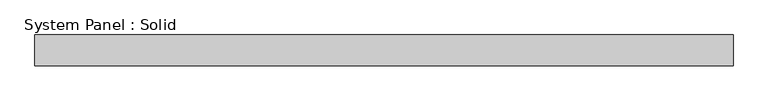
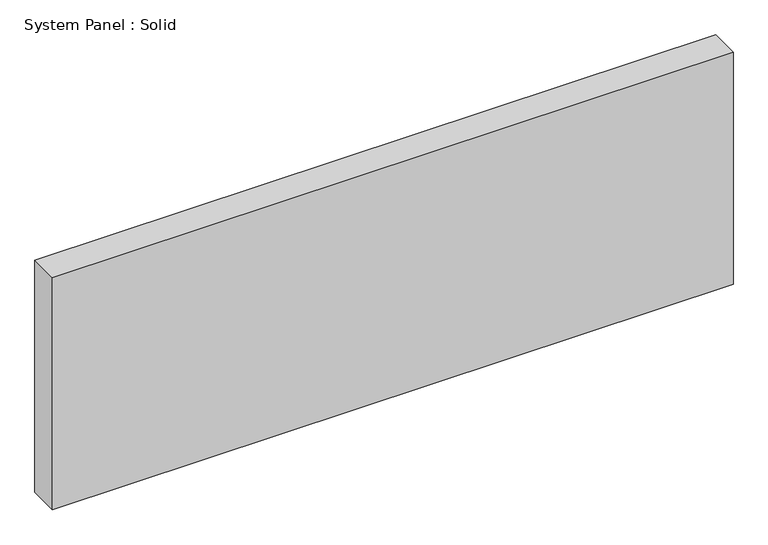
"""IFC4 building model written with IfcOpenShell, lengths in millimetres: plate geometry, System Panel : Solid."""

from ifc_helpers import new_model, si_unit, origin, origin_with_axes, place, context, project, spatial, polyline, outline, extrude, source, transform, mapped, element, save


def system_panel_solid_81598777(model_context):
    return source(origin(), model_context, "Body", "SweptSolid", [
        extrude(outline(polyline([(713.3166666, -44.45), (-713.3166666, -44.45), (-713.3166666, 19.05), (713.3166666, 19.05), (713.3166666, -44.45)])), origin_with_axes(), (0.0, 0.0, 1.0), 514.35),
    ])


if __name__ == "__main__":
    model = new_model("IFC4")
    model_context = context("Model", 3, world=origin())
    ifc_project = project(units=[si_unit("LENGTHUNIT", "METRE", prefix="MILLI")], contexts=[model_context])
    site = spatial("IfcSite", under=ifc_project)
    building = spatial("IfcBuilding", under=site)
    placement = place(None, origin())
    system_panel_solid_shape = system_panel_solid_81598777(model_context)
    element("IfcPlate", 1, ObjectType="System Panel : Solid", at=placement, inside=building, context=model_context, shape_type="MappedRepresentation", body=[
        mapped(system_panel_solid_shape, transform((0.0, 0.0, 0.0), x_axis=(1.0, 0.0, 0.0), y_axis=(0.0, 1.0, 0.0), z_axis=(0.0, 0.0, 1.0))),
    ])
    save(model, "model.ifc")

# Revit data of these elements
# Type "System Panel : Solid"
#   Construction Type Id = "MDOOR"
#   Analytic Construction = "Metal"
#   Visual Light Transmittance = 0
#   Solar Heat Gain Coefficient = 0
#   Heat Transfer Coefficient (U) = 0.651978 BTU/(h·ft²·°F)
#   Define Thermal Properties by = 1
# Element 1 (IfcPlate, "System Panel : Solid")
#   Materials on its faces: "Default"
# Materials
#   "Default": class "Miscellaneous", colour RGB 127 127 127, transparency 0, Cost = 0
